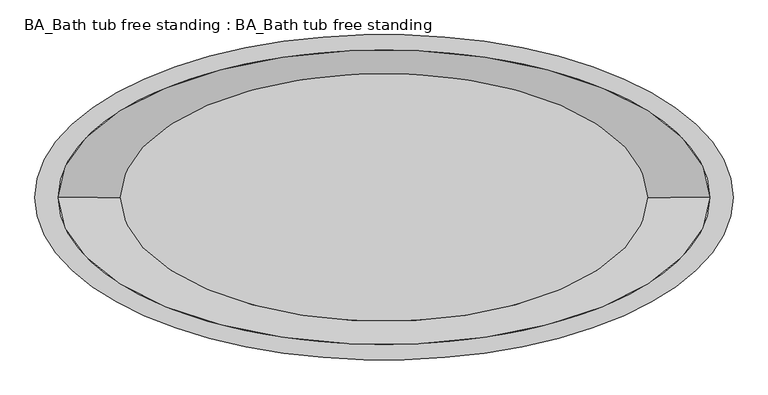
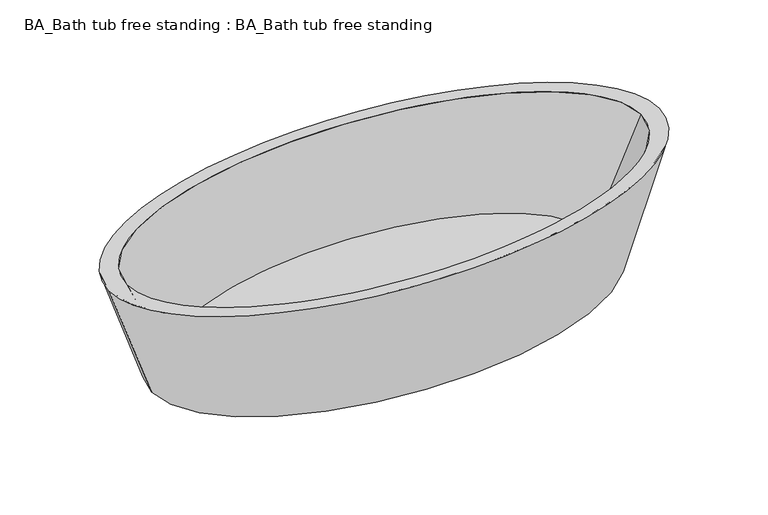
"""IFC4 building model written with IfcOpenShell, lengths in millimetres: flow terminal geometry, BA_Bath tub free standing : BA_Bath tub free standing."""

from ifc_helpers import new_model, si_unit, frame, origin, place, context, project, spatial, ellipse_curve, source, transform, mapped, element, save
from ifc_brep_helpers import plane_surface, spline_surface, advanced_brep


def ba_bath_tub_free_standing_ba_bath_tub_free_standing_c74c3023(model_context):
    return source(origin(), model_context, "Body", "AdvancedBrep", [
        advanced_brep(
        [(900.0, 0.0, 400.0), (-900.0, 0.0, 400.0), (-840.0, 0.0, 400.0), (840.0, 0.0, 400.0), (760.0, 0.0, 0.0), (-760.0, 0.0, 0.0), (680.0, 0.0, 45.9454841), (-680.0, 0.0, 45.9454841)],
        [
            (0, 1, ellipse_curve(frame((0.0, 0.0, 400.0), z_axis=(0.0, 0.0, 1.0), x_axis=(-1.0, 0.0, 0.0)), 900.0, 420.0)),
            (1, 0, ellipse_curve(frame((0.0, 0.0, 400.0), z_axis=(0.0, 0.0, 1.0), x_axis=(-1.0, 0.0, 0.0)), 900.0, 420.0)),
            (2, 3, ellipse_curve(frame((0.0, 0.0, 400.0), z_axis=(0.0, 0.0, -1.0), x_axis=(-1.0, 0.0, 0.0)), 840.0, 380.0)),
            (3, 2, ellipse_curve(frame((0.0, 0.0, 400.0), z_axis=(0.0, 0.0, -1.0), x_axis=(-1.0, 0.0, 0.0)), 840.0, 380.0)),
            (4, 5, ellipse_curve(frame((0.0, 0.0, 0.0), z_axis=(0.0, 0.0, -1.0), x_axis=(-1.0, 0.0, 0.0)), 760.0, 380.0)),
            (5, 4, ellipse_curve(frame((0.0, 0.0, 0.0), z_axis=(0.0, 0.0, -1.0), x_axis=(-1.0, 0.0, 0.0)), 760.0, 380.0)),
            (0, 4),
            (5, 1),
            (6, 7, ellipse_curve(frame((0.0, 0.0, 45.9454841), z_axis=(0.0, 0.0, 1.0), x_axis=(-1.0, 0.0, 0.0)), 680.0, 320.0)),
            (7, 6, ellipse_curve(frame((0.0, 0.0, 45.9454841), z_axis=(0.0, 0.0, 1.0), x_axis=(-1.0, 0.0, 0.0)), 680.0, 320.0)),
            (6, 3),
            (2, 7),
        ],
        [
            plane_surface(frame((0.0, 0.0, 400.0), z_axis=(0.0, 0.0, 1.0), x_axis=(0.0, 1.0, 0.0))),
            plane_surface(frame((0.0, 0.0, 0.0), z_axis=(0.0, 0.0, -1.0), x_axis=(0.0, 1.0, 0.0))),
            spline_surface(2, 1, [[(760.0, 0.0, 0.0), (900.0, 0.0, 400.0)], [(760.0, 380.0, 0.0), (900.0, 420.0, 400.0)], [(0.0, 380.0, 0.0), (0.0, 420.0, 400.0)], [(-760.0, 380.0, 0.0), (-900.0, 420.0, 400.0)], [(-760.0, 0.0, 0.0), (-900.0, 0.0, 400.0)]], [3, 2, 3], [2, 2], [0.0, 1.0, 2.0], [0.0, 1.0], weights=[[1.0, 1.0], [0.7071067811865476, 0.7071067811865476], [1.0, 1.0], [0.7071067811865476, 0.7071067811865476], [1.0, 1.0]]),
            spline_surface(2, 1, [[(-760.0, 0.0, 0.0), (-900.0, 0.0, 400.0)], [(-760.0, -380.0, 0.0), (-900.0, -420.0, 400.0)], [(0.0, -380.0, 0.0), (0.0, -420.0, 400.0)], [(760.0, -380.0, 0.0), (900.0, -420.0, 400.0)], [(760.0, 0.0, 0.0), (900.0, 0.0, 400.0)]], [3, 2, 3], [2, 2], [0.0, 1.0, 2.0], [0.0, 1.0], weights=[[1.0, 1.0], [0.7071067811865476, 0.7071067811865476], [1.0, 1.0], [0.7071067811865476, 0.7071067811865476], [1.0, 1.0]]),
            plane_surface(frame((0.0, 0.0, 45.9454841), z_axis=(0.0, 0.0, 1.0), x_axis=(0.0, 1.0, 0.0))),
            spline_surface(1, 2, [[(680.0, 0.0, 45.9454841), (680.0, 320.0, 45.9454841), (0.0, 320.0, 45.9454841), (-680.0, 320.0, 45.9454841), (-680.0, 0.0, 45.9454841)], [(840.0, 0.0, 400.0), (840.0, 380.0, 400.0), (0.0, 380.0, 400.0), (-840.0, 380.0, 400.0), (-840.0, 0.0, 400.0)]], [2, 2], [3, 2, 3], [0.0, 1.0], [0.0, 1.0, 2.0], weights=[[1.0, 0.7071067811865476, 1.0, 0.7071067811865476, 1.0], [1.0, 0.7071067811865476, 1.0, 0.7071067811865476, 1.0]]),
            spline_surface(1, 2, [[(-680.0, 0.0, 45.9454841), (-680.0, -320.0, 45.9454841), (0.0, -320.0, 45.9454841), (680.0, -320.0, 45.9454841), (680.0, 0.0, 45.9454841)], [(-840.0, 0.0, 400.0), (-840.0, -380.0, 400.0), (0.0, -380.0, 400.0), (840.0, -380.0, 400.0), (840.0, 0.0, 400.0)]], [2, 2], [3, 2, 3], [0.0, 1.0], [0.0, 1.0, 2.0], weights=[[1.0, 0.7071067811865476, 1.0, 0.7071067811865476, 1.0], [1.0, 0.7071067811865476, 1.0, 0.7071067811865476, 1.0]]),
        ],
        [
            (0, [[1, 2], [3, 4]]),
            (1, [[5, 6]]),
            (2, [[-1, 7, -6, 8]]),
            (3, [[-2, -8, -5, -7]]),
            (4, [[9, 10]]),
            (5, [[-9, 11, -3, 12]]),
            (6, [[-10, -12, -4, -11]]),
        ],
    ),
    ])


if __name__ == "__main__":
    model = new_model("IFC4")
    model_context = context("Model", 3, world=origin())
    ifc_project = project(units=[si_unit("LENGTHUNIT", "METRE", prefix="MILLI")], contexts=[model_context])
    site = spatial("IfcSite", under=ifc_project)
    building = spatial("IfcBuilding", under=site)
    placement = place(None, origin())
    ba_bath_tub_free_standing_ba_bath_tub_free_standing_shape = ba_bath_tub_free_standing_ba_bath_tub_free_standing_c74c3023(model_context)
    element("IfcFlowTerminal", 1, ObjectType="BA_Bath tub free standing : BA_Bath tub free standing", at=placement, inside=building, context=model_context, shape_type="MappedRepresentation", body=[
        mapped(ba_bath_tub_free_standing_ba_bath_tub_free_standing_shape, transform((0.0, 0.0, 0.0), x_axis=(1.0, 0.0, 0.0), y_axis=(0.0, 1.0, 0.0), z_axis=(0.0, 0.0, 1.0))),
    ])
    save(model, "model.ifc")

# Revit data of these elements
# Type "BA_Bath tub free standing : BA_Bath tub free standing"
#   Default Elevation = 0
# Element 1 (IfcFlowTerminal, "BA_Bath tub free standing : BA_Bath tub free standing")
#   Materials on its faces: "Default"
# Materials
#   "Default": class "Generic", colour RGB 255 255 255, transparency 0, Cost = 0
